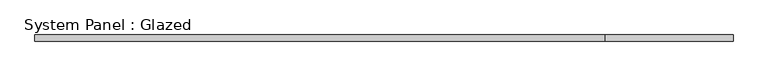
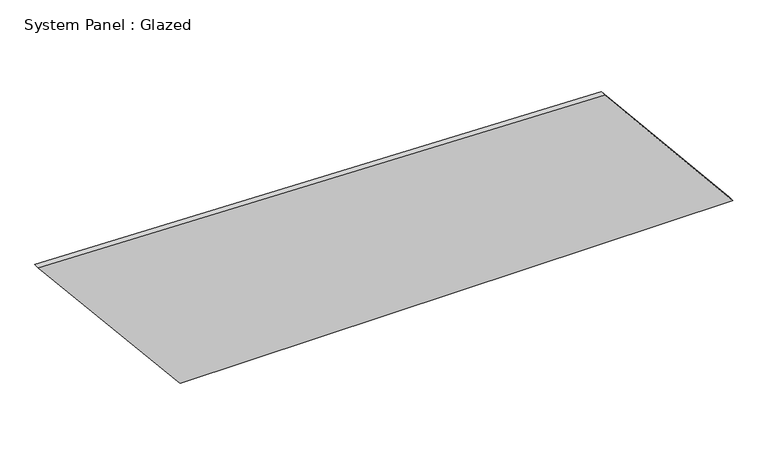
"""IFC4 building model written with IfcOpenShell, lengths in millimetres: plate geometry, System Panel : Glazed."""

from ifc_helpers import new_model, si_unit, frame, origin, place, context, project, spatial, polyline, outline, extrude, source, transform, mapped, element, save


def system_panel_glazed_edcc1857(model_context):
    return source(origin(), model_context, "Body", "SweptSolid", [
        extrude(outline(polyline([(0.0, -839.4265317), (0.0, 1418.9419512), (636.6771589, 896.6160651), (700.1901022, -1418.9419512), (0.0, -839.4265317)])), frame((0.0, -49.5, 0.0), z_axis=(0.0, 1.0, 0.0), x_axis=(0.0, 0.0, 1.0)), (0.0, 0.0, 1.0), 25.0),
    ])


if __name__ == "__main__":
    model = new_model("IFC4")
    model_context = context("Model", 3, world=origin())
    ifc_project = project(units=[si_unit("LENGTHUNIT", "METRE", prefix="MILLI")], contexts=[model_context])
    site = spatial("IfcSite", under=ifc_project)
    building = spatial("IfcBuilding", under=site)
    placement = place(None, origin())
    system_panel_glazed_shape = system_panel_glazed_edcc1857(model_context)
    element("IfcPlate", 1, ObjectType="System Panel : Glazed", at=placement, inside=building, context=model_context, shape_type="MappedRepresentation", body=[
        mapped(system_panel_glazed_shape, transform((0.0, 0.0, 0.0), x_axis=(1.0, 0.0, 0.0), y_axis=(0.0, 1.0, 0.0), z_axis=(0.0, 0.0, 1.0))),
    ])
    save(model, "model.ifc")

# Revit data of these elements
# Element 1 (IfcPlate, "System Panel : Glazed")
#   Materials on its faces: "Glass, Clear Glazing"
# Materials
#   "Glass, Clear Glazing": class "Glass", colour RGB 247 249 248, transparency 0.85, Description = "Clear glazing", Cost = 0
